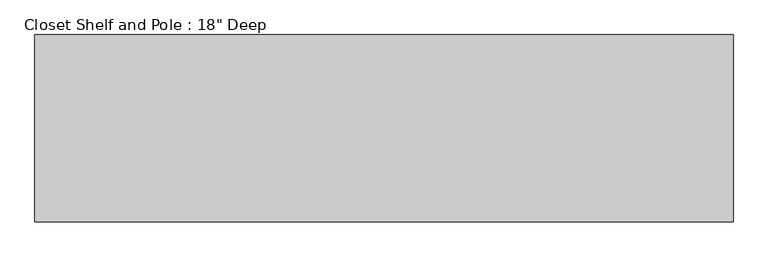
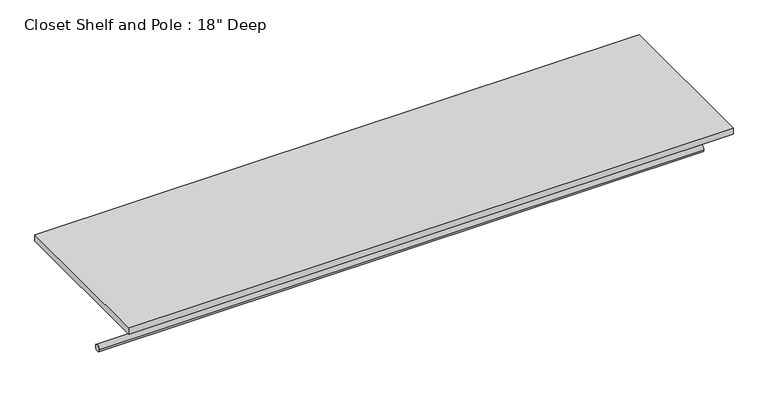
"""IFC4 building model written with IfcOpenShell, lengths in millimetres: proxy geometry."""

from ifc_helpers import new_model, si_unit, point, frame, frame_2d, origin, place, context, project, spatial, polyline, circle_curve, trimmed, segment, composite_curve, outline, extrude, source, transform, mapped, element, save


def proxy_eadc3ce0(model_context):
    return source(origin(), model_context, "Body", "SweptSolid", [
        extrude(outline(composite_curve([segment(trimmed(circle_curve(frame_2d((-304.8, 1676.4)), 9.525), [point((-314.325, 1676.4))], [point((-295.275, 1676.4))], False, "CARTESIAN"), True, "CONTINUOUS"), segment(trimmed(circle_curve(frame_2d((-304.8, 1676.4)), 9.525), [point((-295.275, 1676.4))], [point((-314.325, 1676.4))], False, "CARTESIAN"), True, "CONTINUOUS")], self_intersect=False)), frame((0.0, 0.0, 0.0), z_axis=(1.0, 0.0, 0.0), x_axis=(0.0, 1.0, 0.0)), (0.0, 0.0, 1.0), 1701.8),
        extrude(outline(polyline([(1701.8, 0.0), (1701.8, -457.2), (0.0, -457.2), (0.0, 0.0), (1701.8, 0.0)])), frame((0.0, 0.0, 1809.75), z_axis=(0.0, 0.0, 1.0), x_axis=(1.0, 0.0, 0.0)), (0.0, 0.0, 1.0), 19.05),
    ])


if __name__ == "__main__":
    model = new_model("IFC4")
    model_context = context("Model", 3, world=origin())
    ifc_project = project(units=[si_unit("LENGTHUNIT", "METRE", prefix="MILLI")], contexts=[model_context])
    site = spatial("IfcSite", under=ifc_project)
    building = spatial("IfcBuilding", under=site)
    placement = place(None, origin())
    proxy_shape = proxy_eadc3ce0(model_context)
    element("IfcBuildingElementProxy", 1, Name="Closet Shelf and Pole : 18\" Deep", ObjectType="Closet Shelf and Pole : 18\" Deep", at=placement, inside=building, context=model_context, shape_type="MappedRepresentation", body=[
        mapped(proxy_shape, transform((0.0, 0.0, 0.0), x_axis=(1.0, 0.0, 0.0), y_axis=(0.0, 1.0, 0.0), z_axis=(0.0, 0.0, 1.0))),
    ])
    save(model, "model.ifc")

# Revit data of these elements
# Type "Closet Shelf and Pole : 18\" Deep"
#   Shelf Height = 6' - 0"
#   Depth = 1' - 6"
#   built-in parameter 1001306 [instance default] = 4 (stored number, unit not read)
#   Shelf Material = Birch
#   Default Elevation = 0
# Element 1 (IfcBuildingElementProxy, "Closet Shelf and Pole : 18\" Deep")
#   built-in parameter 1001306 = 5.58333 (stored number, unit not read)
#   Materials on its faces: "Birch"
# Materials
#   "Birch": class "Wood", colour RGB 172 132 95, transparency 0, Description = "Betula Alleghaniensis", Cost = 0
